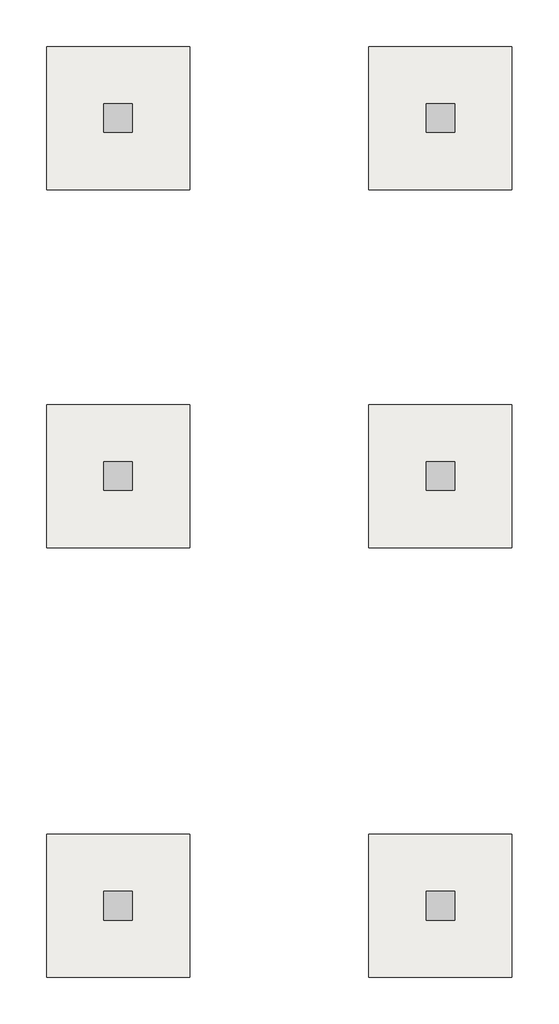
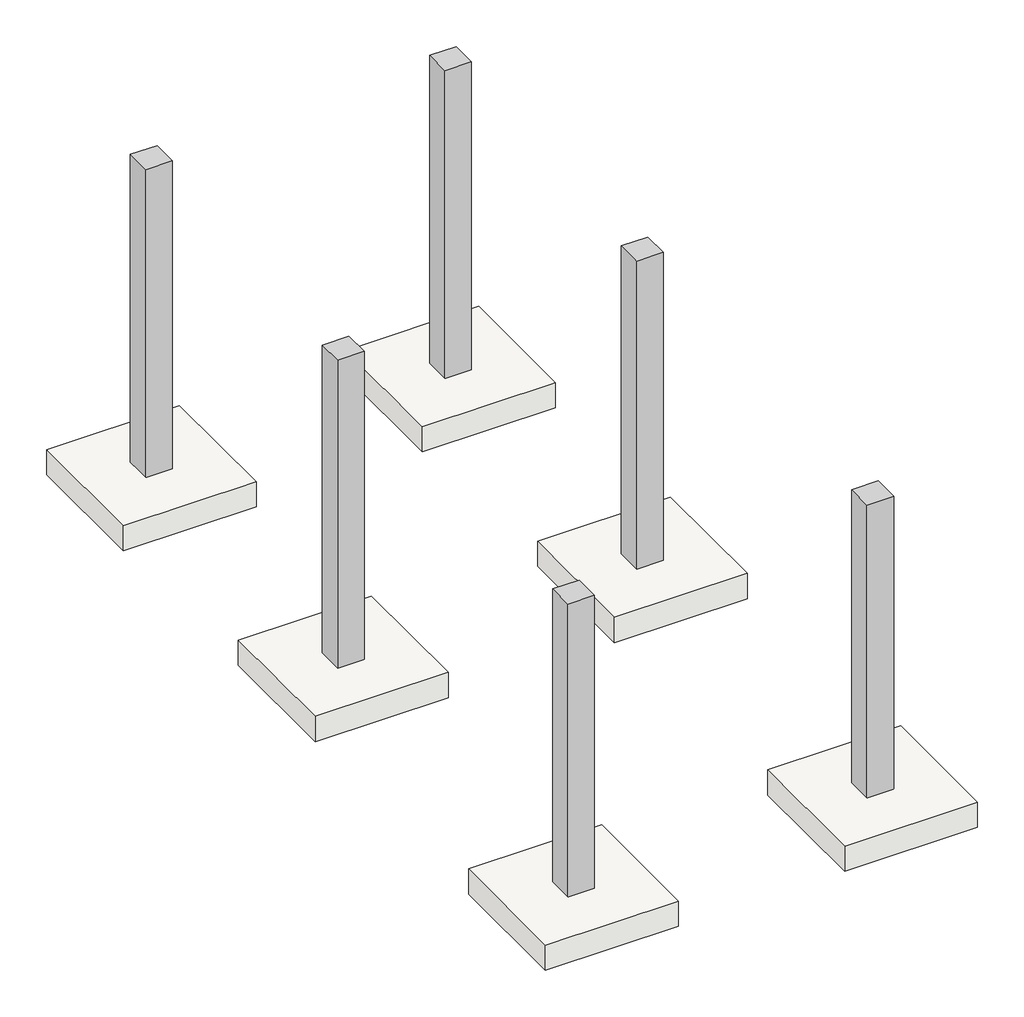
# Not in any storey: 6 columns, 6 slabs.
"""IFC4 building model written with IfcOpenShell, lengths in millimetres."""

import ifcopenshell
import ifcopenshell.guid

model = None  # the IFC model being written
_history = None  # IfcOwnerHistory: only IFC2X3 demands one
_inside = {}  # id of a spatial element -> (the spatial element, [elements in it])
_under = {}  # id of a project, library or spatial element -> (it, [spatial elements below it])
_declared = {}  # id of a project -> (the project, [libraries it declares])
_typed = {}  # id of a type object -> (the type object, [elements of that type])
_made_of = {}  # id of a material, layer set ... -> (it, [elements and type objects made of it])


def new_model(schema):
    """Start an empty IFC model of exactly this schema.

    Asked for "IFC4X3", IfcOpenShell would pick the latest addendum, in which some entities
    have other attributes; the version numbers below select the first issue.
    IFC2X3 requires an IfcOwnerHistory on every rooted entity: one is made here for all.
    """
    global model, _history
    if schema == "IFC4X3":
        model = ifcopenshell.file(schema_version=(4, 3, 0, 0))
    else:
        model = ifcopenshell.file(schema=schema)
    _inside.clear()
    _under.clear()
    _declared.clear()
    _typed.clear()
    _made_of.clear()
    _history = None
    if model.schema == "IFC2X3":
        org = make("IfcOrganization", Name="unknown")
        user = make(
            "IfcPersonAndOrganization",
            ThePerson=make("IfcPerson", FamilyName="unknown"),
            TheOrganization=org,
        )
        app = make(
            "IfcApplication",
            ApplicationDeveloper=org,
            Version="unknown",
            ApplicationFullName="unknown",
            ApplicationIdentifier="unknown",
        )
        _history = make(
            "IfcOwnerHistory",
            OwningUser=user,
            OwningApplication=app,
            ChangeAction="ADDED",
            CreationDate=0,
        )
    return model


def make(cls, **values):
    """One entity of the class cls with the attributes given. An attribute that is None is left unset."""
    return model.create_entity(
        cls, **{name: value for name, value in values.items() if value is not None}
    )


def rooted(cls, **values):
    """An entity with a GlobalId (a new one), such as an element, a storey or a relation."""
    return make(cls, GlobalId=ifcopenshell.guid.new(), OwnerHistory=_history, **values)


def si_unit(unit_type, name, prefix=None):
    """IfcSIUnit, for example si_unit("LENGTHUNIT", "METRE", prefix="MILLI")."""
    return make("IfcSIUnit", UnitType=unit_type, Prefix=prefix, Name=name)


def assignment(units):
    """IfcUnitAssignment: the units of a project."""
    return None if units is None else make("IfcUnitAssignment", Units=units)


def point(xyz):
    """IfcCartesianPoint."""
    return None if xyz is None else make("IfcCartesianPoint", Coordinates=xyz)


def direction(xyz):
    """IfcDirection."""
    return None if xyz is None else make("IfcDirection", DirectionRatios=xyz)


def frame(location, z_axis=None, x_axis=None):
    """IfcAxis2Placement3D, a coordinate frame: its origin and axes. An axis left out is left unset."""
    return make(
        "IfcAxis2Placement3D",
        Location=point(location),
        Axis=direction(z_axis),
        RefDirection=direction(x_axis),
    )


def origin():
    """The frame at (0, 0, 0) with its axes left unset."""
    return frame((0.0, 0.0, 0.0))


def place(relative_to, where):
    """IfcLocalPlacement: puts the frame where relative to a parent placement (None: the world)."""
    return make(
        "IfcLocalPlacement", PlacementRelTo=relative_to, RelativePlacement=where
    )


def context(
    kind, dimensions, precision=None, world=None, true_north=None, identifier=None
):
    """IfcGeometricRepresentationContext, for example the 3D "Model" context."""
    return make(
        "IfcGeometricRepresentationContext",
        ContextIdentifier=identifier,
        ContextType=kind,
        CoordinateSpaceDimension=dimensions,
        Precision=precision,
        WorldCoordinateSystem=world,
        TrueNorth=true_north,
    )


def project(units=None, contexts=None):
    """IfcProject with its units and contexts."""
    return rooted(
        "IfcProject",
        Name="project",
        RepresentationContexts=contexts,
        UnitsInContext=assignment(units),
    )


def spatial(cls, under=None, at=None, **own):
    """A site, building, storey or space (cls), placed at a placement, below another one or the project."""
    s = rooted(cls, ObjectPlacement=at, **own)
    if under is not None:
        _under.setdefault(under.id(), (under, []))[1].append(s)
    return s


def polyline(points):
    """IfcPolyline through the points."""
    return make("IfcPolyline", Points=[point(p) for p in points])


def outline(outer, holes=None, kind="AREA"):
    """IfcArbitraryClosedProfileDef: a profile drawn as a closed curve; with holes, ...WithVoids."""
    if holes is None:
        return make("IfcArbitraryClosedProfileDef", ProfileType=kind, OuterCurve=outer)
    return make(
        "IfcArbitraryProfileDefWithVoids",
        ProfileType=kind,
        OuterCurve=outer,
        InnerCurves=holes,
    )


def extrude(swept, where, along, depth):
    """IfcExtrudedAreaSolid: the profile swept, set in the frame where, extruded along a direction by depth."""
    return make(
        "IfcExtrudedAreaSolid",
        SweptArea=swept,
        Position=where,
        ExtrudedDirection=direction(along),
        Depth=depth,
    )


def faces_of(points, faces, orient=None, outer=None):
    """IfcFace entities. A face is a list of loops; a loop is a list of indices into points, from 0.

    orient and outer hold one flag for each loop. By default every Orientation is true, the
    first loop of a face is its IfcFaceOuterBound and the others are IfcFaceBound.
    """
    made = []
    for i, loops in enumerate(faces):
        bounds = []
        for j, loop in enumerate(loops):
            is_outer = j == 0 if outer is None else outer[i][j]
            bounds.append(
                make(
                    "IfcFaceOuterBound" if is_outer else "IfcFaceBound",
                    Bound=make("IfcPolyLoop", Polygon=[points[k] for k in loop]),
                    Orientation=True if orient is None else orient[i][j],
                )
            )
        made.append(make("IfcFace", Bounds=bounds))
    return made


def faceted_brep(points, faces, orient=None, outer=None, voids=None):
    """IfcFacetedBrep: a solid bounded by flat faces; with voids (closed shells), ...WithVoids."""
    shared = [point(p) for p in points]
    hull = make("IfcClosedShell", CfsFaces=faces_of(shared, faces, orient, outer))
    if voids is None:
        return make("IfcFacetedBrep", Outer=hull)
    return make(
        "IfcFacetedBrepWithVoids",
        Outer=hull,
        Voids=[
            make(cls, CfsFaces=faces_of(shared, fs, o, b)) for cls, fs, o, b in voids
        ],
    )


def shape(context_of_items, identifier, shape_type, items):
    """IfcShapeRepresentation: the items that make up one representation, for example the "Body"."""
    return make(
        "IfcShapeRepresentation",
        ContextOfItems=context_of_items,
        RepresentationIdentifier=identifier,
        RepresentationType=shape_type,
        Items=items,
    )


def source(mapping_origin, context_of_items, identifier, shape_type, items):
    """IfcRepresentationMap: a shape defined once, which mapped items show again and again."""
    return make(
        "IfcRepresentationMap",
        MappingOrigin=mapping_origin,
        MappedRepresentation=shape(context_of_items, identifier, shape_type, items),
    )


def transform(
    local_origin,
    x_axis=None,
    y_axis=None,
    z_axis=None,
    scale=None,
    scale2=None,
    scale3=None,
    uniform=True,
):
    """IfcCartesianTransformationOperator3D, or its non-uniform kind. x_axis, y_axis, z_axis: its Axis1, 2, 3."""
    if uniform:
        return make(
            "IfcCartesianTransformationOperator3D",
            Axis1=direction(x_axis),
            Axis2=direction(y_axis),
            LocalOrigin=point(local_origin),
            Scale=scale,
            Axis3=direction(z_axis),
        )
    return make(
        "IfcCartesianTransformationOperator3DnonUniform",
        Axis1=direction(x_axis),
        Axis2=direction(y_axis),
        LocalOrigin=point(local_origin),
        Scale=scale,
        Axis3=direction(z_axis),
        Scale2=scale2,
        Scale3=scale3,
    )


def mapped(mapping_source, mapping_target):
    """IfcMappedItem: shows the shape of a source again, moved by a transform."""
    return make(
        "IfcMappedItem", MappingSource=mapping_source, MappingTarget=mapping_target
    )


def made_of(thing, what):
    """Note that an element or type object is made of a material, layer set ...; save() writes the relation."""
    if what is not None:
        _made_of.setdefault(what.id(), (what, []))[1].append(thing)
    return thing


def element(
    cls,
    number,
    at=None,
    inside=None,
    cuts=None,
    type_object=None,
    material=None,
    context=None,
    identifier="Body",
    shape_type=None,
    held_by="IfcProductDefinitionShape",
    body=None,
    shapes=None,
    **own,
):
    """One element of the class cls, such as IfcWall. Its Tag is "e" and its number.

    at: its placement. inside: the storey or other place that contains it. cuts: it is an
    opening in that element (IfcRelVoidsElement). A single representation is given by context,
    identifier, shape_type and body (its items); several are given by shapes. held_by: the class
    of the entity that holds the representations. save() writes the other relations.
    """
    e = rooted(cls, Tag="e%d" % number, ObjectPlacement=at, **own)
    if body is not None:
        shapes = [shape(context, identifier, shape_type, body)]
    if shapes is not None:
        e.Representation = make(held_by, Representations=shapes)
    if inside is not None:
        _inside.setdefault(inside.id(), (inside, []))[1].append(e)
    if cuts is not None:
        rooted(
            "IfcRelVoidsElement", RelatingBuildingElement=cuts, RelatedOpeningElement=e
        )
    if type_object is not None:
        _typed.setdefault(type_object.id(), (type_object, []))[1].append(e)
    return made_of(e, material)


def aggregate(whole, parts):
    """IfcRelAggregates: a whole, such as a stair, and the parts it consists of."""
    return rooted("IfcRelAggregates", RelatingObject=whole, RelatedObjects=parts)


def save(model, path):
    """Write the relations noted so far, then the file.

    IfcRelAggregates (storeys below a building ...), IfcRelContainedInSpatialStructure (elements
    in a storey), IfcRelDefinesByType, IfcRelAssociatesMaterial and IfcRelDeclares: one each for
    every whole, place, type object, material and project.
    """
    for whole, parts in _under.values():
        aggregate(whole, parts)
    for where, things in _inside.values():
        rooted(
            "IfcRelContainedInSpatialStructure",
            RelatedElements=things,
            RelatingStructure=where,
        )
    for kind, things in _typed.values():
        rooted("IfcRelDefinesByType", RelatedObjects=things, RelatingType=kind)
    for what, things in _made_of.values():
        rooted("IfcRelAssociatesMaterial", RelatedObjects=things, RelatingMaterial=what)
    for by, libraries in _declared.values():
        rooted("IfcRelDeclares", RelatingContext=by, RelatedDefinitions=libraries)
    model.write(path)


def ft211_footing_rectangular_r1_4779d05c(model_context):
    return source(origin(), model_context, "Body", "SweptSolid", [
        extrude(outline(polyline([(1000.0, 1000.0), (1000.0, -1000.0), (-1000.0, -1000.0), (-1000.0, 1000.0), (1000.0, 1000.0)])), frame((0.0, 0.0, -400.0), z_axis=(0.0, 0.0, 1.0), x_axis=(1.0, 0.0, 0.0)), (0.0, 0.0, 1.0), 400.0),
    ])


model = new_model("IFC4")

# Units and contexts
model_context = context("Model", 3, world=origin())
ifc_project = project(units=[si_unit("LENGTHUNIT", "METRE", prefix="MILLI")], contexts=[model_context])

# Site, building
site = spatial("IfcSite", under=ifc_project)
building = spatial("IfcBuilding", under=site)

# Columns
placement = place(None, origin())
element("IfcColumn", 1, ObjectType="RC_Column_Rectangular : H_SC_ACC_W400xL400", at=placement, inside=building, context=model_context, shape_type="Brep", body=[
    faceted_brep([(-1563.0, 9960.0208589, 198500.0), (-1563.0, 9560.0208589, 198500.0), (-1963.0, 9560.0208589, 198500.0), (-1963.0, 9960.0208589, 198500.0), (-1563.0, 9960.0208589, 203400.0), (-1563.0, 9560.0208589, 203400.0), (-1563.0, 9560.0208589, 202750.0), (-1563.0, 9960.0208589, 202750.0), (-1963.0, 9560.0208589, 203400.0), (-1963.0, 9960.0208589, 203400.0)], [[[0, 1, 2, 3]], [[4, 5, 6, 1, 0, 7]], [[5, 8, 2, 1, 6]], [[8, 9, 3, 2]], [[9, 4, 7, 0, 3]], [[4, 9, 8, 5]]]),
])
element("IfcColumn", 2, ObjectType="RC_Column_Rectangular : H_SC_ACC_W400xL400", at=placement, inside=building, context=model_context, shape_type="Brep", body=[
    faceted_brep([(2937.0, 9960.0208589, 198500.0), (2937.0, 9560.0208589, 198500.0), (2537.0, 9560.0208589, 198500.0), (2537.0, 9960.0208589, 198500.0), (2937.0, 9960.0208589, 203400.0), (2937.0, 9560.0208589, 203400.0), (2937.0, 9560.0208589, 202750.0), (2937.0, 9560.0208589, 200250.0), (2937.0, 9560.0208589, 199650.0), (2537.0, 9560.0208589, 203400.0), (2537.0, 9560.0208589, 202750.0), (2537.0, 9560.0208589, 200250.0), (2537.0, 9560.0208589, 199650.0), (2537.0, 9960.0208589, 203400.0), (2537.0, 9960.0208589, 202750.0)], [[[0, 1, 2, 3]], [[4, 5, 6, 7, 8, 1, 0]], [[5, 9, 10, 11, 12, 2, 1, 8, 7, 6]], [[9, 13, 14, 3, 2, 12, 11, 10]], [[13, 4, 0, 3, 14]], [[4, 13, 9, 5]]]),
])
element("IfcColumn", 3, ObjectType="RC_Column_Rectangular : H_SC_ACC_W400xL400", at=placement, inside=building, context=model_context, shape_type="Brep", body=[
    faceted_brep([(-1563.0, -1039.9791411, 198500.0), (-1563.0, -1439.9791411, 198500.0), (-1963.0, -1439.9791411, 198500.0), (-1963.0, -1039.9791411, 198500.0), (-1563.0, -1039.9791411, 203160.0), (-1563.0, -1439.9791411, 203160.0), (-1563.0, -1439.9791411, 200250.0), (-1563.0, -1439.9791411, 199650.0), (-1563.0, -1039.9791411, 199650.0), (-1563.0, -1039.9791411, 200250.0), (-1963.0, -1439.9791411, 203160.0), (-1963.0, -1039.9791411, 203160.0), (-1963.0, -1039.9791411, 200250.0), (-1963.0, -1039.9791411, 199650.0)], [[[0, 1, 2, 3]], [[4, 5, 6, 7, 1, 0, 8, 9]], [[5, 10, 2, 1, 7, 6]], [[10, 11, 12, 13, 3, 2]], [[11, 4, 9, 8, 0, 3, 13, 12]], [[4, 11, 10, 5]]]),
])
element("IfcColumn", 4, ObjectType="RC_Column_Rectangular : H_SC_ACC_W400xL400", at=placement, inside=building, context=model_context, shape_type="Brep", body=[
    faceted_brep([(2937.0, -1039.9791411, 198500.0), (2937.0, -1439.9791411, 198500.0), (2537.0, -1439.9791411, 198500.0), (2537.0, -1039.9791411, 198500.0), (2937.0, -1039.9791411, 203160.0), (2937.0, -1439.9791411, 203160.0), (2937.0, -1039.9791411, 199650.0), (2937.0, -1039.9791411, 200250.0), (2537.0, -1439.9791411, 203160.0), (2537.0, -1439.9791411, 200250.0), (2537.0, -1439.9791411, 199650.0), (2537.0, -1039.9791411, 203160.0), (2537.0, -1039.9791411, 200250.0), (2537.0, -1039.9791411, 199650.0)], [[[0, 1, 2, 3]], [[4, 5, 1, 0, 6, 7]], [[5, 8, 9, 10, 2, 1]], [[8, 11, 12, 13, 3, 2, 10, 9]], [[11, 4, 7, 6, 0, 3, 13, 12]], [[4, 11, 8, 5]]]),
])
element("IfcColumn", 5, ObjectType="RC_Column_Rectangular : H_SC_ACC_W400xL400", at=placement, inside=building, context=model_context, shape_type="Brep", body=[
    faceted_brep([(-1563.0, 4960.0208589, 198500.0), (-1563.0, 4560.0208589, 198500.0), (-1963.0, 4560.0208589, 198500.0), (-1963.0, 4960.0208589, 198500.0), (-1563.0, 4960.0208589, 203400.0), (-1563.0, 4560.0208589, 203400.0), (-1563.0, 4560.0208589, 202750.0), (-1563.0, 4560.0208589, 200250.0), (-1563.0, 4560.0208589, 199650.0), (-1563.0, 4960.0208589, 199650.0), (-1563.0, 4960.0208589, 200250.0), (-1563.0, 4960.0208589, 202750.0), (-1963.0, 4560.0208589, 203400.0), (-1963.0, 4560.0208589, 200250.0), (-1963.0, 4560.0208589, 199650.0), (-1963.0, 4960.0208589, 203400.0), (-1963.0, 4960.0208589, 202750.0), (-1963.0, 4960.0208589, 200250.0), (-1963.0, 4960.0208589, 199650.0)], [[[0, 1, 2, 3]], [[4, 5, 6, 7, 8, 1, 0, 9, 10, 11]], [[5, 12, 13, 14, 2, 1, 8, 7, 6]], [[12, 15, 16, 17, 18, 3, 2, 14, 13]], [[15, 4, 11, 10, 9, 0, 3, 18, 17, 16]], [[4, 15, 12, 5]]]),
])
element("IfcColumn", 6, ObjectType="RC_Column_Rectangular : H_SC_ACC_W400xL400", at=placement, inside=building, context=model_context, shape_type="Brep", body=[
    faceted_brep([(2937.0, 4960.0208589, 198500.0), (2937.0, 4560.0208589, 198500.0), (2537.0, 4560.0208589, 198500.0), (2537.0, 4960.0208589, 198500.0), (2937.0, 4960.0208589, 203400.0), (2937.0, 4560.0208589, 203400.0), (2937.0, 4560.0208589, 200250.0), (2937.0, 4560.0208589, 199650.0), (2937.0, 4960.0208589, 199650.0), (2937.0, 4960.0208589, 200250.0), (2937.0, 4960.0208589, 202750.0), (2537.0, 4560.0208589, 203400.0), (2537.0, 4560.0208589, 202750.0), (2537.0, 4560.0208589, 200250.0), (2537.0, 4560.0208589, 199650.0), (2537.0, 4960.0208589, 203400.0), (2537.0, 4960.0208589, 202750.0), (2537.0, 4960.0208589, 200250.0), (2537.0, 4960.0208589, 199650.0)], [[[0, 1, 2, 3]], [[4, 5, 6, 7, 1, 0, 8, 9, 10]], [[5, 11, 12, 13, 14, 2, 1, 7, 6]], [[11, 15, 16, 17, 18, 3, 2, 14, 13, 12]], [[15, 4, 10, 9, 8, 0, 3, 18, 17, 16]], [[4, 15, 11, 5]]]),
])

# Slabs
ft211_footing_rectangular_r1_shape = ft211_footing_rectangular_r1_4779d05c(model_context)
element("IfcSlab", 7, ObjectType="FT211-Footing-Rectangular_R1 : H_SF_ACF_W2000xL2000xT400_Bitumen", at=placement, inside=building, context=model_context, shape_type="MappedRepresentation", body=[
    mapped(ft211_footing_rectangular_r1_shape, transform((-1763.0, 9760.0208589, 198500.0), x_axis=(1.0, 0.0, 0.0), y_axis=(0.0, 1.0, 0.0), z_axis=(0.0, 0.0, 1.0))),
])
element("IfcSlab", 8, ObjectType="FT211-Footing-Rectangular_R1 : H_SF_ACF_W2000xL2000xT400_Bitumen", at=placement, inside=building, context=model_context, shape_type="MappedRepresentation", body=[
    mapped(ft211_footing_rectangular_r1_shape, transform((2737.0, 9760.0208589, 198500.0), x_axis=(1.0, 0.0, 0.0), y_axis=(0.0, 1.0, 0.0), z_axis=(0.0, 0.0, 1.0))),
])
element("IfcSlab", 9, ObjectType="FT211-Footing-Rectangular_R1 : H_SF_ACF_W2000xL2000xT400_Bitumen", at=placement, inside=building, context=model_context, shape_type="MappedRepresentation", body=[
    mapped(ft211_footing_rectangular_r1_shape, transform((-1763.0, -1239.9791411, 198500.0), x_axis=(1.0, 0.0, 0.0), y_axis=(0.0, 1.0, 0.0), z_axis=(0.0, 0.0, 1.0))),
])
element("IfcSlab", 10, ObjectType="FT211-Footing-Rectangular_R1 : H_SF_ACF_W2000xL2000xT400_Bitumen", at=placement, inside=building, context=model_context, shape_type="MappedRepresentation", body=[
    mapped(ft211_footing_rectangular_r1_shape, transform((2737.0, -1239.9791411, 198500.0), x_axis=(1.0, 0.0, 0.0), y_axis=(0.0, 1.0, 0.0), z_axis=(0.0, 0.0, 1.0))),
])
element("IfcSlab", 11, ObjectType="FT211-Footing-Rectangular_R1 : H_SF_ACF_W2000xL2000xT400_Bitumen", at=placement, inside=building, context=model_context, shape_type="MappedRepresentation", body=[
    mapped(ft211_footing_rectangular_r1_shape, transform((-1763.0, 4760.0208589, 198500.0), x_axis=(1.0, 0.0, 0.0), y_axis=(0.0, 1.0, 0.0), z_axis=(0.0, 0.0, 1.0))),
])
element("IfcSlab", 12, ObjectType="FT211-Footing-Rectangular_R1 : H_SF_ACF_W2000xL2000xT400_Bitumen", at=placement, inside=building, context=model_context, shape_type="MappedRepresentation", body=[
    mapped(ft211_footing_rectangular_r1_shape, transform((2737.0, 4760.0208589, 198500.0), x_axis=(1.0, 0.0, 0.0), y_axis=(0.0, 1.0, 0.0), z_axis=(0.0, 0.0, 1.0))),
])

save(model, "model.ifc")

# Revit data of these elements
# Type "RC_Column_Rectangular : H_SC_ACC_W400xL400"
#   Width = 400.000 mm
#   Length = 400.000 mm
#   hec_material3 [instance default] = none
#   hec_material2 [instance default] = none
#   hec_material1 [instance default] = none
#   Structural Material [instance default] = none
#   Description = (empty or 0)
# Type "FT211-Footing-Rectangular_R1 : H_SF_ACF_W2000xL2000xT400_Bitumen"
#   Top bar = "D25@300"
#   Description = "UG Shallow Foundation"
#   Bottom bar = "D20@300"
#   Width = 2000.000 mm
#   Length = 2000.000 mm
#   Foundation Thickness = 400.000 mm
#   Structural Material [instance default] = none
#   Assembly Code = ""
# Elements 1, 2, 3, 4, 5, 6 (IfcColumn, "RC_Column_Rectangular : H_SC_ACC_W400xL400")
#   Comments = ""
#   hec_material3 = none
#   hec_material2 = none
#   hec_material1 = none
#   Structural Material = none
#   Phase Created = New Construction
# Elements 7, 8, 9, 10, 11, 12 (IfcSlab, "FT211-Footing-Rectangular_R1 : H_SF_ACF_W2000xL2000xT400_Bitumen")
#   Comments = ""
#   Structural Material = none
#   Phase Created = New Construction
